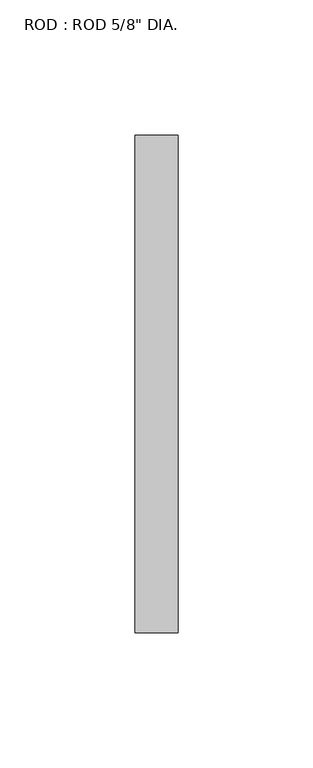
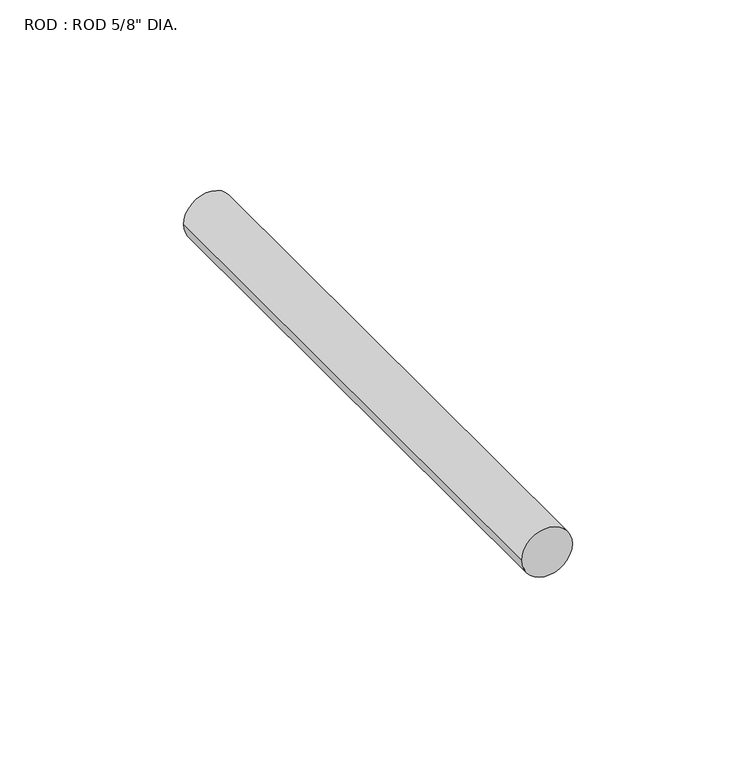
"""IFC4 building model written with IfcOpenShell, lengths in millimetres: proxy geometry."""

from ifc_helpers import new_model, si_unit, point, frame, origin, origin_2d, place, context, project, spatial, circle_curve, trimmed, segment, composite_curve, outline, extrude, source, transform, mapped, element, save


def proxy_1bf62e37(model_context):
    return source(origin(), model_context, "Body", "SweptSolid", [
        extrude(outline(composite_curve([segment(trimmed(circle_curve(origin_2d(), 7.9375), [point((0.0, 7.9375))], [point((0.0, -7.9375))], False, "CARTESIAN"), True, "CONTINUOUS"), segment(trimmed(circle_curve(origin_2d(), 7.9375), [point((0.0, -7.9375))], [point((0.0, 7.9375))], False, "CARTESIAN"), True, "CONTINUOUS")], self_intersect=False)), frame((0.0, -152.4, 0.0), z_axis=(0.0, 1.0, 0.0), x_axis=(0.0, 0.0, 1.0)), (0.0, 0.0, 1.0), 184.15),
    ])


if __name__ == "__main__":
    model = new_model("IFC4")
    model_context = context("Model", 3, world=origin())
    ifc_project = project(units=[si_unit("LENGTHUNIT", "METRE", prefix="MILLI")], contexts=[model_context])
    site = spatial("IfcSite", under=ifc_project)
    building = spatial("IfcBuilding", under=site)
    placement = place(None, origin())
    proxy_shape = proxy_1bf62e37(model_context)
    element("IfcBuildingElementProxy", 1, Name="ROD : ROD 5/8\" DIA.", ObjectType="ROD : ROD 5/8\" DIA.", at=placement, inside=building, context=model_context, shape_type="MappedRepresentation", body=[
        mapped(proxy_shape, transform((0.0, 0.0, 0.0), x_axis=(1.0, 0.0, 0.0), y_axis=(0.0, 1.0, 0.0), z_axis=(0.0, 0.0, 1.0))),
    ])
    save(model, "model.ifc")

# Revit data of these elements
# Type "ROD : ROD 5/8\" DIA."
#   lenght = 0' - 7 1/4"
#   Radius = 0' - 0 5/16"
#   material [instance default] = 3/4" GALV. THRU BOLTS
# Materials
#   "3/4\" GALV. THRU BOLTS": class "Generic", colour RGB 105 69 171, transparency 0, Cost = 0
